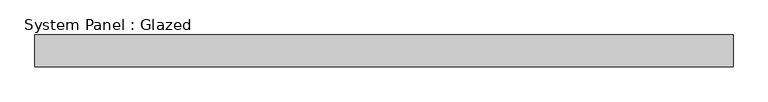
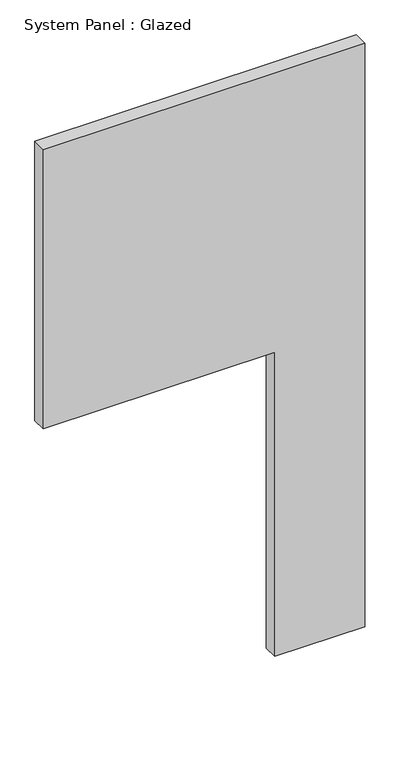
"""IFC4 building model written with IfcOpenShell, lengths in millimetres: plate geometry, System Panel : Glazed."""

from ifc_helpers import new_model, si_unit, frame, origin, place, context, project, spatial, polyline, outline, extrude, source, transform, mapped, element, save


def system_panel_glazed_05ea4a17(model_context):
    return source(origin(), model_context, "Body", "SweptSolid", [
        extrude(outline(polyline([(0.0, 241.8930392), (0.0, 550.0006382), (2110.0, 550.0006382), (2110.0, -550.0006382), (1100.0, -550.0006382), (1100.0, 241.8930392), (0.0, 241.8930392)])), frame((0.0, -25.0, 0.0), z_axis=(0.0, 1.0, 0.0), x_axis=(0.0, 0.0, 1.0)), (0.0, 0.0, 1.0), 50.0),
    ])


if __name__ == "__main__":
    model = new_model("IFC4")
    model_context = context("Model", 3, world=origin())
    ifc_project = project(units=[si_unit("LENGTHUNIT", "METRE", prefix="MILLI")], contexts=[model_context])
    site = spatial("IfcSite", under=ifc_project)
    building = spatial("IfcBuilding", under=site)
    placement = place(None, origin())
    system_panel_glazed_shape = system_panel_glazed_05ea4a17(model_context)
    element("IfcPlate", 1, ObjectType="System Panel : Glazed", at=placement, inside=building, context=model_context, shape_type="MappedRepresentation", body=[
        mapped(system_panel_glazed_shape, transform((0.0, 0.0, 0.0), x_axis=(1.0, 0.0, 0.0), y_axis=(0.0, 1.0, 0.0), z_axis=(0.0, 0.0, 1.0))),
    ])
    save(model, "model.ifc")

# Revit data of these elements
# Type "System Panel : Glazed"
#   Type Mark = "CW-GLASS"
# Element 1 (IfcPlate, "System Panel : Glazed")
#   Materials on its faces: "Glass_Clear"
# Materials
#   "Glass_Clear": class "Glass", colour RGB 128 128 255, transparency 0.8, Comments = "Rendering appearance not upgraded ", Cost = 0
